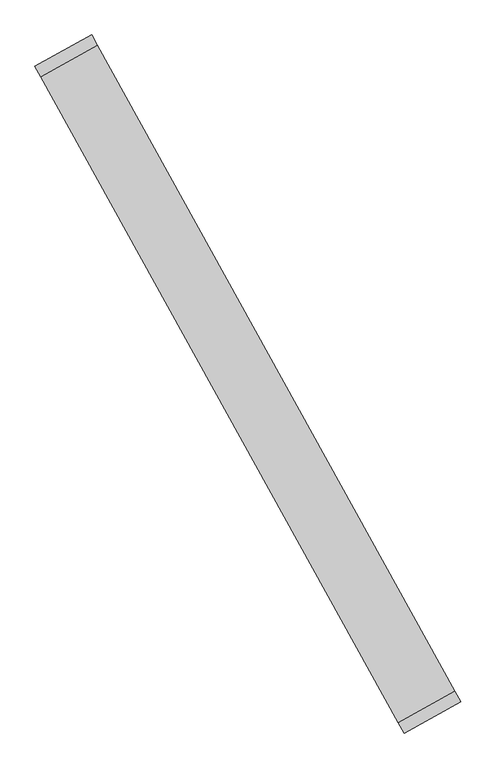
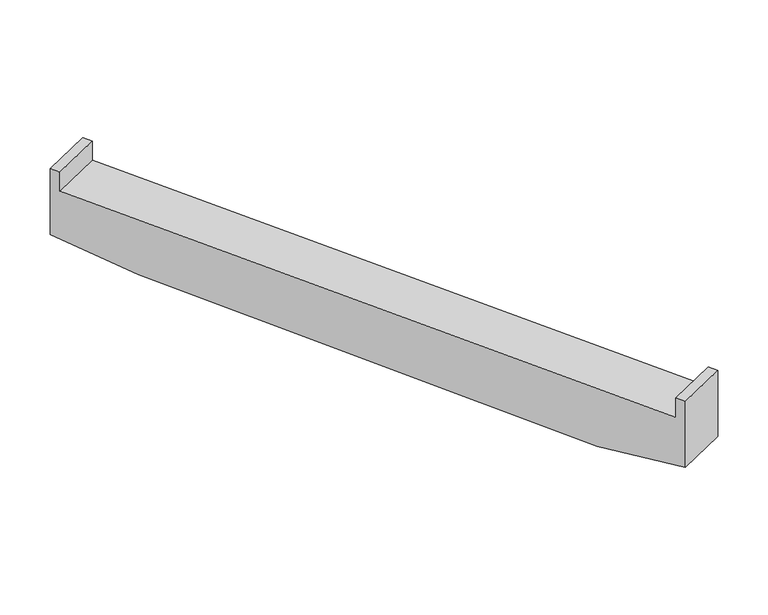
"""IFC4 building model written with IfcOpenShell, lengths in millimetres: beam geometry, KNA_SF_Tussensteunpunt As1 : KNA_SF_Tussensteunpunt As2."""

from ifc_helpers import new_model, si_unit, frame, origin, place, context, project, spatial, polyline, outline, extrude, source, transform, mapped, element, save


def beam_e4c7b040(model_context):
    return source(origin(), model_context, "Body", "SweptSolid", [
        extrude(outline(polyline([(300.0, 0.0), (300.0, -200.0), (-1110.0, -200.0), (-1310.0, 1600.0), (-1604.360945, 10952.6559729), (-1404.360945, 12752.6559728), (5.639055, 12752.6559728), (5.639055, 12552.6559728), (-405.5480197, 12552.6559728), (-108.8635701, 0.0), (300.0, 0.0)])), frame((130211.1374129, -37808.197421, 4379.040393), z_axis=(0.8748782267130669, 0.4843429450538115, 0.0), x_axis=(0.0, 0.0, 1.0)), (0.0, 0.0, 1.0), 1100.0),
    ])


if __name__ == "__main__":
    model = new_model("IFC4")
    model_context = context("Model", 3, world=origin())
    ifc_project = project(units=[si_unit("LENGTHUNIT", "METRE", prefix="MILLI")], contexts=[model_context])
    site = spatial("IfcSite", under=ifc_project)
    building = spatial("IfcBuilding", under=site)
    placement = place(None, origin())
    beam_shape = beam_e4c7b040(model_context)
    element("IfcBeam", 1, ObjectType="KNA_SF_Tussensteunpunt As1 : KNA_SF_Tussensteunpunt As2", at=placement, inside=building, context=model_context, shape_type="MappedRepresentation", body=[
        mapped(beam_shape, transform((0.0, 0.0, 0.0), x_axis=(1.0, 0.0, 0.0), y_axis=(0.0, 1.0, 0.0), z_axis=(0.0, 0.0, 1.0))),
    ])
    save(model, "model.ifc")
